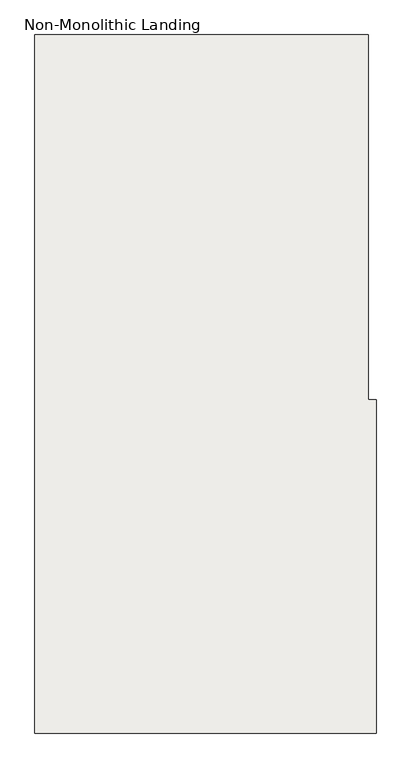
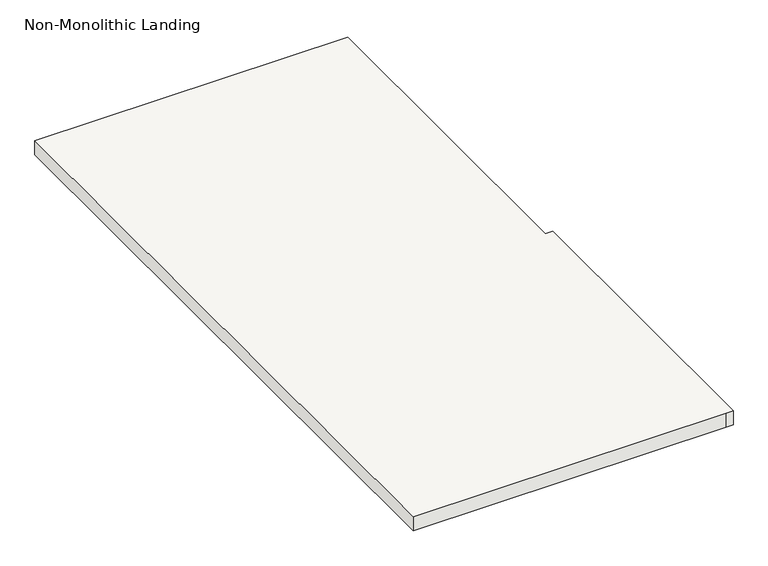
"""IFC4 building model written with IfcOpenShell, lengths in millimetres: slab geometry, Non-Monolithic Landing."""

from ifc_helpers import new_model, si_unit, origin, place, context, project, spatial, faceted_brep, source, transform, mapped, element, save


def non_monolithic_landing_895fb0ff(model_context):
    return source(origin(), model_context, "Body", "Brep", [
        faceted_brep([(663695.788677, -549416.0413841, 2179.7662162), (663721.188677, -549416.0413841, 2205.1662162), (663721.188677, -550482.8413841, 2205.1662162), (663695.788677, -550482.8413841, 2179.7662162), (662654.388677, -549416.0413841, 2224.2162162), (662654.388677, -551651.2413841, 2224.2162162), (663721.188677, -551651.2413841, 2224.2162162), (663746.588677, -551651.2413841, 2224.2162162), (663746.588677, -550584.4413841, 2224.2162162), (663721.188677, -550584.4413841, 2224.2162162), (663721.188677, -549416.0413841, 2224.2162162), (663695.788677, -550482.8413841, 2173.4162162), (663721.188677, -550482.8413841, 2173.4162162), (663721.188677, -550584.4413841, 2173.4162162), (663746.588677, -550584.4413841, 2173.4162162), (663746.588677, -551651.2413841, 2173.4162162), (663721.188677, -551651.2413841, 2173.4162162), (662654.388677, -551651.2413841, 2173.4162162), (662654.388677, -549416.0413841, 2173.4162162), (663695.788677, -549416.0413841, 2173.4162162)], [[[0, 1, 2, 3]], [[4, 5, 6, 7, 8, 9, 10]], [[11, 12, 13, 14, 15, 16, 17, 18, 19]], [[12, 11, 3, 2]], [[11, 19, 0, 3]], [[4, 10, 1, 0, 19, 18]], [[5, 4, 18, 17]], [[6, 5, 17, 16]], [[7, 6, 16, 15]], [[8, 7, 15, 14]], [[9, 8, 14, 13]], [[10, 9, 13, 12, 2, 1]]]),
    ])


if __name__ == "__main__":
    model = new_model("IFC4")
    model_context = context("Model", 3, world=origin())
    ifc_project = project(units=[si_unit("LENGTHUNIT", "METRE", prefix="MILLI")], contexts=[model_context])
    site = spatial("IfcSite", under=ifc_project)
    building = spatial("IfcBuilding", under=site)
    placement = place(None, origin())
    non_monolithic_landing_shape = non_monolithic_landing_895fb0ff(model_context)
    element("IfcSlab", 1, ObjectType="Non-Monolithic Landing", at=placement, inside=building, context=model_context, shape_type="MappedRepresentation", body=[
        mapped(non_monolithic_landing_shape, transform((0.0, 0.0, 0.0), x_axis=(1.0, 0.0, 0.0), y_axis=(0.0, 1.0, 0.0), z_axis=(0.0, 0.0, 1.0))),
    ])
    save(model, "model.ifc")
